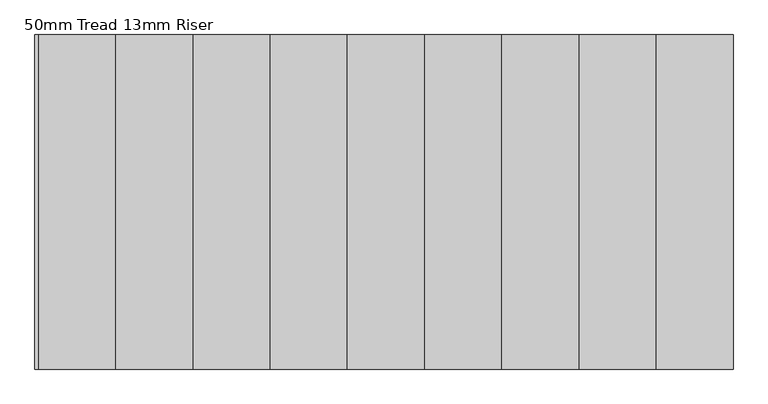
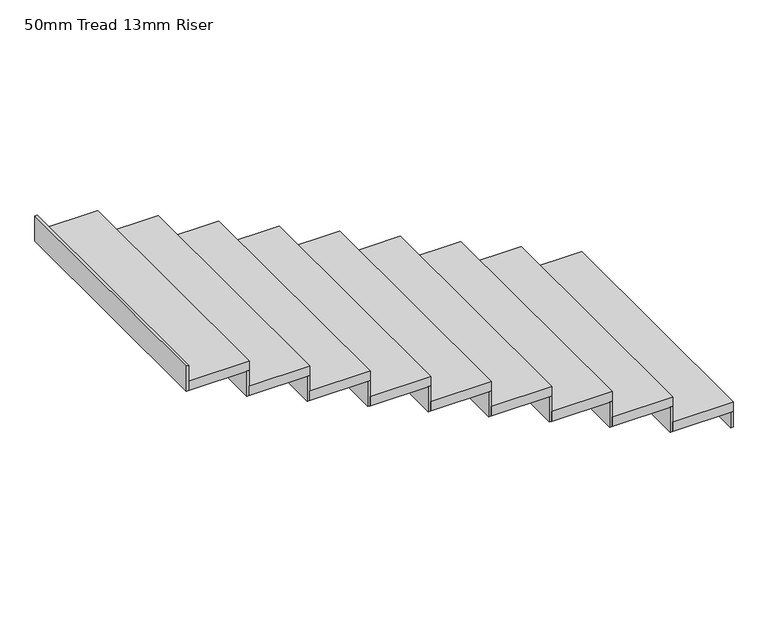
"""IFC4 building model written with IfcOpenShell, lengths in millimetres: stair flight geometry, 50mm Tread 13mm Riser."""

from ifc_helpers import new_model, si_unit, frame, origin, place, context, project, spatial, polyline, outline, extrude, source, transform, mapped, element, save


def stair_flight_50mm_tread_13mm_riser_9679e67a(model_context):
    return source(origin(), model_context, "Body", "SweptSolid", [
        extrude(outline(polyline([(-10508.0859635, -1819.3642494), (-10495.5859635, -1819.3642494), (-10495.5859635, -3119.3642494), (-10508.0859635, -3119.3642494), (-10508.0859635, -1819.3642494)])), frame((0.0, 0.0, 3000.0), z_axis=(0.0, 0.0, 1.0), x_axis=(1.0, 0.0, 0.0)), (0.0, 0.0, 1.0), 82.0),
        extrude(outline(polyline([(-10795.5859635, -3119.3642494), (-10795.5859635, -1819.3642494), (-10495.5859635, -1819.3642494), (-10495.5859635, -3119.3642494), (-10795.5859635, -3119.3642494)])), frame((0.0, 0.0, 3082.0), z_axis=(0.0, 0.0, 1.0), x_axis=(1.0, 0.0, 0.0)), (0.0, 0.0, 1.0), 50.0),
        extrude(outline(polyline([(-10808.0859635, -1819.3642494), (-10795.5859635, -1819.3642494), (-10795.5859635, -3119.3642494), (-10808.0859635, -3119.3642494), (-10808.0859635, -1819.3642494)])), frame((0.0, 0.0, 3082.0), z_axis=(0.0, 0.0, 1.0), x_axis=(1.0, 0.0, 0.0)), (0.0, 0.0, 1.0), 132.0),
        extrude(outline(polyline([(-11095.5859635, -3119.3642494), (-11095.5859635, -1819.3642494), (-10795.5859635, -1819.3642494), (-10795.5859635, -3119.3642494), (-11095.5859635, -3119.3642494)])), frame((0.0, 0.0, 3214.0), z_axis=(0.0, 0.0, 1.0), x_axis=(1.0, 0.0, 0.0)), (0.0, 0.0, 1.0), 50.0),
        extrude(outline(polyline([(-11108.0859635, -1819.3642494), (-11095.5859635, -1819.3642494), (-11095.5859635, -3119.3642494), (-11108.0859635, -3119.3642494), (-11108.0859635, -1819.3642494)])), frame((0.0, 0.0, 3214.0), z_axis=(0.0, 0.0, 1.0), x_axis=(1.0, 0.0, 0.0)), (0.0, 0.0, 1.0), 132.0),
        extrude(outline(polyline([(-11395.5859635, -3119.3642494), (-11395.5859635, -1819.3642494), (-11095.5859635, -1819.3642494), (-11095.5859635, -3119.3642494), (-11395.5859635, -3119.3642494)])), frame((0.0, 0.0, 3346.0), z_axis=(0.0, 0.0, 1.0), x_axis=(1.0, 0.0, 0.0)), (0.0, 0.0, 1.0), 50.0),
        extrude(outline(polyline([(-11408.0859635, -1819.3642494), (-11395.5859635, -1819.3642494), (-11395.5859635, -3119.3642494), (-11408.0859635, -3119.3642494), (-11408.0859635, -1819.3642494)])), frame((0.0, 0.0, 3346.0), z_axis=(0.0, 0.0, 1.0), x_axis=(1.0, 0.0, 0.0)), (0.0, 0.0, 1.0), 132.0),
        extrude(outline(polyline([(-11695.5859635, -3119.3642494), (-11695.5859635, -1819.3642494), (-11395.5859635, -1819.3642494), (-11395.5859635, -3119.3642494), (-11695.5859635, -3119.3642494)])), frame((0.0, 0.0, 3478.0), z_axis=(0.0, 0.0, 1.0), x_axis=(1.0, 0.0, 0.0)), (0.0, 0.0, 1.0), 50.0),
        extrude(outline(polyline([(-11708.0859635, -1819.3642494), (-11695.5859635, -1819.3642494), (-11695.5859635, -3119.3642494), (-11708.0859635, -3119.3642494), (-11708.0859635, -1819.3642494)])), frame((0.0, 0.0, 3478.0), z_axis=(0.0, 0.0, 1.0), x_axis=(1.0, 0.0, 0.0)), (0.0, 0.0, 1.0), 132.0),
        extrude(outline(polyline([(-11995.5859635, -3119.3642494), (-11995.5859635, -1819.3642494), (-11695.5859635, -1819.3642494), (-11695.5859635, -3119.3642494), (-11995.5859635, -3119.3642494)])), frame((0.0, 0.0, 3610.0), z_axis=(0.0, 0.0, 1.0), x_axis=(1.0, 0.0, 0.0)), (0.0, 0.0, 1.0), 50.0),
        extrude(outline(polyline([(-12008.0859635, -1819.3642494), (-11995.5859635, -1819.3642494), (-11995.5859635, -3119.3642494), (-12008.0859635, -3119.3642494), (-12008.0859635, -1819.3642494)])), frame((0.0, 0.0, 3610.0), z_axis=(0.0, 0.0, 1.0), x_axis=(1.0, 0.0, 0.0)), (0.0, 0.0, 1.0), 132.0),
        extrude(outline(polyline([(-12295.5859635, -3119.3642494), (-12295.5859635, -1819.3642494), (-11995.5859635, -1819.3642494), (-11995.5859635, -3119.3642494), (-12295.5859635, -3119.3642494)])), frame((0.0, 0.0, 3742.0), z_axis=(0.0, 0.0, 1.0), x_axis=(1.0, 0.0, 0.0)), (0.0, 0.0, 1.0), 50.0),
        extrude(outline(polyline([(-12308.0859635, -1819.3642494), (-12295.5859635, -1819.3642494), (-12295.5859635, -3119.3642494), (-12308.0859635, -3119.3642494), (-12308.0859635, -1819.3642494)])), frame((0.0, 0.0, 3742.0), z_axis=(0.0, 0.0, 1.0), x_axis=(1.0, 0.0, 0.0)), (0.0, 0.0, 1.0), 132.0),
        extrude(outline(polyline([(-12595.5859635, -3119.3642494), (-12595.5859635, -1819.3642494), (-12295.5859635, -1819.3642494), (-12295.5859635, -3119.3642494), (-12595.5859635, -3119.3642494)])), frame((0.0, 0.0, 3874.0), z_axis=(0.0, 0.0, 1.0), x_axis=(1.0, 0.0, 0.0)), (0.0, 0.0, 1.0), 50.0),
        extrude(outline(polyline([(-12608.0859635, -1819.3642494), (-12595.5859635, -1819.3642494), (-12595.5859635, -3119.3642494), (-12608.0859635, -3119.3642494), (-12608.0859635, -1819.3642494)])), frame((0.0, 0.0, 3874.0), z_axis=(0.0, 0.0, 1.0), x_axis=(1.0, 0.0, 0.0)), (0.0, 0.0, 1.0), 132.0),
        extrude(outline(polyline([(-12895.5859635, -3119.3642494), (-12895.5859635, -1819.3642494), (-12595.5859635, -1819.3642494), (-12595.5859635, -3119.3642494), (-12895.5859635, -3119.3642494)])), frame((0.0, 0.0, 4006.0), z_axis=(0.0, 0.0, 1.0), x_axis=(1.0, 0.0, 0.0)), (0.0, 0.0, 1.0), 50.0),
        extrude(outline(polyline([(-12908.0859635, -1819.3642494), (-12895.5859635, -1819.3642494), (-12895.5859635, -3119.3642494), (-12908.0859635, -3119.3642494), (-12908.0859635, -1819.3642494)])), frame((0.0, 0.0, 4006.0), z_axis=(0.0, 0.0, 1.0), x_axis=(1.0, 0.0, 0.0)), (0.0, 0.0, 1.0), 132.0),
        extrude(outline(polyline([(-13208.0859635, -1819.3642494), (-13195.5859635, -1819.3642494), (-13195.5859635, -3119.3642494), (-13208.0859635, -3119.3642494), (-13208.0859635, -1819.3642494)])), frame((0.0, 0.0, 4138.0), z_axis=(0.0, 0.0, 1.0), x_axis=(1.0, 0.0, 0.0)), (0.0, 0.0, 1.0), 132.0),
        extrude(outline(polyline([(-13195.5859635, -3119.3642494), (-13195.5859635, -1819.3642494), (-12895.5859635, -1819.3642494), (-12895.5859635, -3119.3642494), (-13195.5859635, -3119.3642494)])), frame((0.0, 0.0, 4138.0), z_axis=(0.0, 0.0, 1.0), x_axis=(1.0, 0.0, 0.0)), (0.0, 0.0, 1.0), 50.0),
    ])


if __name__ == "__main__":
    model = new_model("IFC4")
    model_context = context("Model", 3, world=origin())
    ifc_project = project(units=[si_unit("LENGTHUNIT", "METRE", prefix="MILLI")], contexts=[model_context])
    site = spatial("IfcSite", under=ifc_project)
    building = spatial("IfcBuilding", under=site)
    placement = place(None, origin())
    stair_flight_50mm_tread_13mm_riser_shape = stair_flight_50mm_tread_13mm_riser_9679e67a(model_context)
    element("IfcStairFlight", 1, ObjectType="50mm Tread 13mm Riser", at=placement, inside=building, context=model_context, shape_type="MappedRepresentation", body=[
        mapped(stair_flight_50mm_tread_13mm_riser_shape, transform((0.0, 0.0, 0.0), x_axis=(1.0, 0.0, 0.0), y_axis=(0.0, 1.0, 0.0), z_axis=(0.0, 0.0, 1.0))),
    ])
    save(model, "model.ifc")
